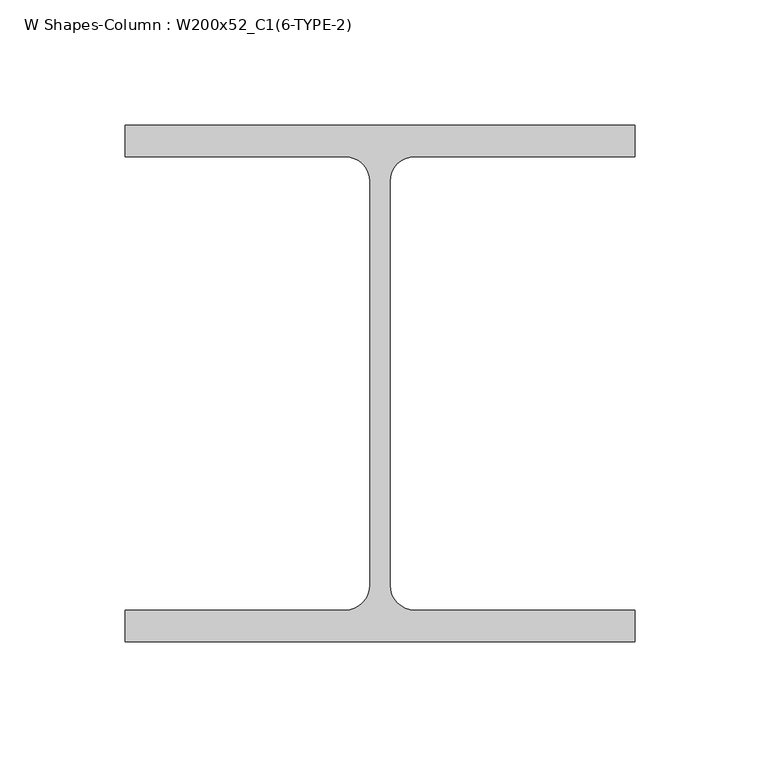
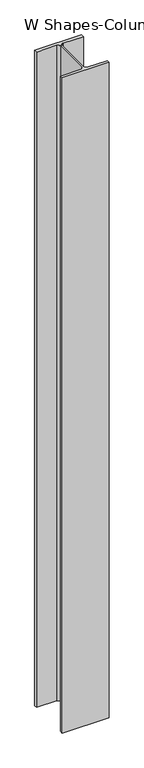
"""IFC4 building model written with IfcOpenShell, lengths in millimetres: column geometry, W Shapes-Column : W200x52_C1(6-TYPE-2)."""

from ifc_helpers import new_model, si_unit, point, frame, frame_2d, origin, place, context, project, spatial, polyline, circle_curve, trimmed, segment, composite_curve, outline, extrude, source, transform, mapped, element, save


def w_shapes_column_w200x52_c1_6_type_2_67715140(model_context):
    return source(origin(), model_context, "Body", "SweptSolid", [
        extrude(outline(composite_curve([segment(polyline([(101.854, -103.124), (-101.854, -103.124), (-101.854, -90.551), (-13.9446, -90.551)]), True, "CONTINUOUS"), segment(trimmed(circle_curve(frame_2d((-13.9446, -80.5434)), 10.0076), [point((-13.9446, -90.551))], [point((-3.937, -80.5434))], True, "CARTESIAN"), True, "CONTINUOUS"), segment(polyline([(-3.937, -80.5434), (-3.937, 80.5434)]), True, "CONTINUOUS"), segment(trimmed(circle_curve(frame_2d((-13.9446, 80.5434)), 10.0076), [point((-3.937, 80.5434))], [point((-13.9446, 90.551))], True, "CARTESIAN"), True, "CONTINUOUS"), segment(polyline([(-13.9446, 90.551), (-101.854, 90.551), (-101.854, 103.124), (101.854, 103.124), (101.854, 90.551), (13.9446, 90.551)]), True, "CONTINUOUS"), segment(trimmed(circle_curve(frame_2d((13.9446, 80.5434)), 10.0076), [point((13.9446, 90.551))], [point((3.937, 80.5434))], True, "CARTESIAN"), True, "CONTINUOUS"), segment(polyline([(3.937, 80.5434), (3.937, -80.5434)]), True, "CONTINUOUS"), segment(trimmed(circle_curve(frame_2d((13.9446, -80.5434)), 10.0076), [point((3.937, -80.5434))], [point((13.9446, -90.551))], True, "CARTESIAN"), True, "CONTINUOUS"), segment(polyline([(13.9446, -90.551), (101.854, -90.551), (101.854, -103.124)]), True, "CONTINUOUS")], self_intersect=False)), frame((0.0, 0.0, 9760.0), z_axis=(0.0, 0.0, 1.0), x_axis=(1.0, 0.0, 0.0)), (0.0, 0.0, 1.0), 3000.0),
    ])


if __name__ == "__main__":
    model = new_model("IFC4")
    model_context = context("Model", 3, world=origin())
    ifc_project = project(units=[si_unit("LENGTHUNIT", "METRE", prefix="MILLI")], contexts=[model_context])
    site = spatial("IfcSite", under=ifc_project)
    building = spatial("IfcBuilding", under=site)
    placement = place(None, origin())
    w_shapes_column_w200x52_c1_6_type_2_shape = w_shapes_column_w200x52_c1_6_type_2_67715140(model_context)
    element("IfcColumn", 1, ObjectType="W Shapes-Column : W200x52_C1(6-TYPE-2)", at=placement, inside=building, context=model_context, shape_type="MappedRepresentation", body=[
        mapped(w_shapes_column_w200x52_c1_6_type_2_shape, transform((0.0, 0.0, 0.0), x_axis=(1.0, 0.0, 0.0), y_axis=(0.0, 1.0, 0.0), z_axis=(0.0, 0.0, 1.0))),
    ])
    save(model, "model.ifc")

# Revit data of these elements
# Type "W Shapes-Column : W200x52_C1(6-TYPE-2)"
#   Section Name Key = "W8X35"
#   Assembly Code = "B10"
#   Width = 20.3708 cm
#   Web Thickness = 0.7874 cm
#   Web Fillet = 1.0008 cm
#   Warping Constant = 166223.7 cm⁶
#   Torsional Moment of Inertia = 32.0082 cm⁴
#   Section Area = 66.4515 cm²
#   Plastic Modulus weak axis = 263.832 cm³
#   Plastic Modulus strong axis = 568.631 cm³
#   Perimeter = 1.1936 m²/m
#   Nominal Weight = 52.0857 kgf/m
#   Moment of Inertia weak axis = 1773.15 cm⁴
#   Moment of Inertia strong axis = 5286.14 cm⁴
#   Height = 20.6248 cm
#   Flange Thickness = 1.2573 cm
#   Elastic Modulus weak axis = 173.703 cm³
#   Elastic Modulus strong axis = 511.276 cm³
#   Clear Web Height = 14.605 cm
#   Centroid Vertical = 10.3124 cm
#   Centroid Horizontal = 10.1854 cm
#   Bolt Spacing = 13.97 cm
#   Structural Material [instance default] = Steel ASTM A992
#   Principal Axes Angle = 0
# Element 1 (IfcColumn, "W Shapes-Column : W200x52_C1(6-TYPE-2)")
#   Structural Material = none
# Materials
#   "Steel ASTM A992": class "Metal", colour RGB 199 199 199, transparency 0, Description = "Structural steel 50ksi", Cost = 0
